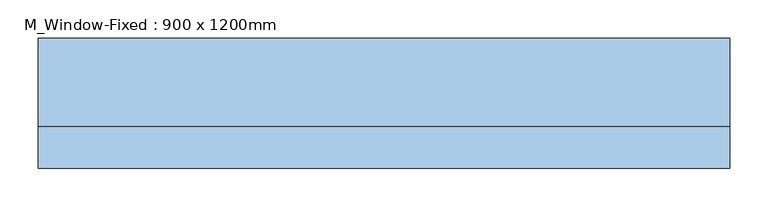
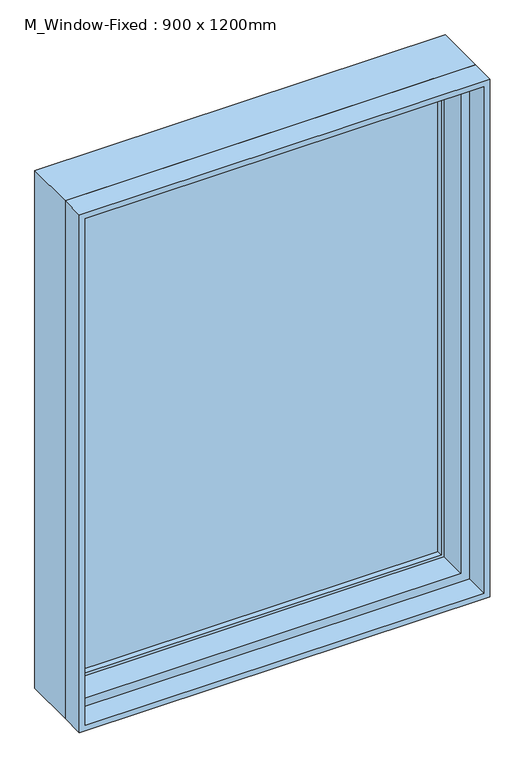
"""IFC4 building model written with IfcOpenShell, lengths in millimetres: window geometry, M_Window-Fixed : 900 x 1200mm."""

from ifc_helpers import new_model, si_unit, frame, origin, place, context, project, spatial, polyline, outline, extrude, faceted_brep, source, transform, mapped, element, save


def m_window_fixed_900_x_1200mm_f2c8dc95(model_context):
    return source(origin(), model_context, "Body", "SolidModel", [
        faceted_brep([(450.0, -20.25, 2100.0), (450.0, 94.05, 2100.0), (-450.0, 94.05, 2100.0), (-450.0, -20.25, 2100.0), (-450.0, 94.05, 900.0), (-450.0, -20.25, 900.0), (450.0, 94.05, 900.0), (450.0, -20.25, 900.0), (418.25, -20.25, 2068.25), (418.25, -20.25, 931.75), (-418.25, -20.25, 931.75), (-418.25, -20.25, 2068.25), (-437.3, 94.05, 2087.3), (-437.3, 94.05, 912.7), (437.3, 94.05, 912.7), (437.3, 94.05, 2087.3), (418.25, 43.25, 2068.25), (-418.25, 43.25, 2068.25), (437.3, 43.25, 2087.3), (-437.3, 43.25, 2087.3), (-418.25, 43.25, 931.75), (-437.3, 43.25, 912.7), (418.25, 43.25, 931.75), (437.3, 43.25, 912.7)], [[[0, 1, 2, 3]], [[3, 2, 4, 5]], [[5, 4, 6, 7]], [[3, 5, 7, 0], [8, 9, 10, 11]], [[7, 6, 1, 0]], [[1, 6, 4, 2], [12, 13, 14, 15]], [[16, 8, 11, 17]], [[15, 18, 19, 12]], [[17, 11, 10, 20]], [[12, 19, 21, 13]], [[20, 10, 9, 22]], [[13, 21, 23, 14]], [[22, 9, 8, 16]], [[18, 23, 21, 19], [17, 20, 22, 16]], [[14, 23, 18, 15]]]),
        extrude(outline(polyline([(2100.0, -450.0), (900.0, -450.0), (900.0, 450.0), (2100.0, 450.0), (2100.0, -450.0)]), holes=[polyline([(2087.3, 437.3), (912.7, 437.3), (912.7, -437.3), (2087.3, -437.3), (2087.3, 437.3)])]), frame((0.0, -75.0, 0.0), z_axis=(0.0, 1.0, 0.0), x_axis=(0.0, 0.0, 1.0)), (0.0, 0.0, 1.0), 54.75),
        extrude(outline(polyline([(912.7, 437.3), (2087.3, 437.3), (2087.3, -437.3), (912.7, -437.3), (912.7, 437.3)]), holes=[polyline([(938.1, -411.9), (2061.9, -411.9), (2061.9, 411.9), (938.1, 411.9), (938.1, -411.9)])]), frame((0.0, 43.25, 0.0), z_axis=(0.0, 1.0, 0.0), x_axis=(0.0, 0.0, 1.0)), (0.0, 0.0, 1.0), 44.45),
        extrude(outline(polyline([(411.9, 75.0), (411.9, 68.65), (-411.9, 68.65), (-411.9, 75.0), (411.9, 75.0)])), frame((0.0, 0.0, 938.1), z_axis=(0.0, 0.0, 1.0), x_axis=(1.0, 0.0, 0.0)), (0.0, 0.0, 1.0), 1123.8),
        extrude(outline(polyline([(-411.9, 55.95), (-411.9, 62.3), (411.9, 62.3), (411.9, 55.95), (-411.9, 55.95)])), frame((0.0, 0.0, 938.1), z_axis=(0.0, 0.0, 1.0), x_axis=(1.0, 0.0, 0.0)), (0.0, 0.0, 1.0), 1123.8),
    ])


if __name__ == "__main__":
    model = new_model("IFC4")
    model_context = context("Model", 3, world=origin())
    ifc_project = project(units=[si_unit("LENGTHUNIT", "METRE", prefix="MILLI")], contexts=[model_context])
    site = spatial("IfcSite", under=ifc_project)
    building = spatial("IfcBuilding", under=site)
    placement = place(None, origin())
    m_window_fixed_900_x_1200mm_shape = m_window_fixed_900_x_1200mm_f2c8dc95(model_context)
    element("IfcWindow", 1, ObjectType="M_Window-Fixed : 900 x 1200mm", at=placement, inside=building, context=model_context, shape_type="MappedRepresentation", body=[
        mapped(m_window_fixed_900_x_1200mm_shape, transform((0.0, 0.0, 0.0), x_axis=(1.0, 0.0, 0.0), y_axis=(0.0, 1.0, 0.0), z_axis=(0.0, 0.0, 1.0))),
    ])
    save(model, "model.ifc")

# Revit data of these elements
# Type "M_Window-Fixed : 900 x 1200mm"
#   Type Mark = "36"
#   Fire Rating = "0.5h"
#   Analytic Construction = "Double glazing - domestic"
#   Window Inset [instance default] = 0 mm
#   Wall Thickness [instance default] = 150 mm
#   Visual Light Transmittance = 0.81
#   Thermal Resistance (R) = 0.319569 (m²·K)/W
#   Solar Heat Gain Coefficient = 0.76
#   Rough Width = 915 mm
#   Rough Height = 1215 mm
#   Interior Wall Closure [instance default] = 54.75 mm
#   Height = 1200 mm
#   Heat Transfer Coefficient (U) = 3.12929 W/(m²·K)
#   Frame Extension [instance default] = 6.35 mm
#   Exterior Wall Closure [instance default] = 31.75 mm
#   Extension Jamb [instance default] = 54.75 mm
#   Default Sill Height = 900 mm
#   Width = 900 mm
#   Muntin Visibility = yes
#   Interior Trim Visibility [instance default] = yes
#   Exterior Trim Visibility [instance default] = yes
#   Extension Jamb Visibility [instance default] = yes
#   Muntin Pattern = M_Muntin Pattern_2x2 : M_Muntin Pattern_2x2
#   Interior Trim Material = Wood - Stained
#   Interior Trim = M_Trim-Window-Interior-Flat : Picture Frame
#   Interior Frame Material = Wood - Stained
#   Glass Panel Material = Glass
#   Exterior Trim Material = Clad - White
#   Exterior Trim = M_Trim-Window-Exterior-Flat : with Sill
#   Exterior Frame Material = Clad - White
#   Wall Closure = (empty or 0)
# Element 1 (IfcWindow, "M_Window-Fixed : 900 x 1200mm")
#   Materials on its faces: "Wood - Stained", "Glass", "Clad - White"
# Materials
#   "Wood - Stained": class "Wood", colour RGB 173 132 96, transparency 0, Cost = 0
#   "Glass": class "Glass", colour RGB 245 245 243, transparency 1, Description = "Soda Lime Glass", Cost = 0
#   "Clad - White": class "Wood", colour RGB 245 245 243, transparency 0, Cost = 0
